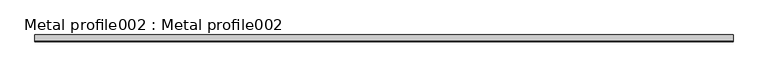
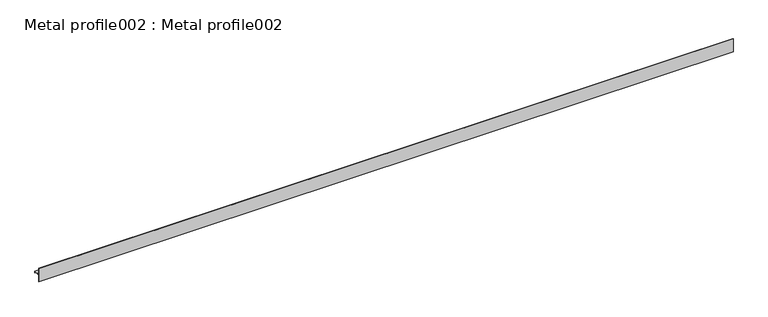
"""IFC4 building model written with IfcOpenShell, lengths in millimetres: proxy geometry, Metal profile002 : Metal profile002."""

from ifc_helpers import new_model, si_unit, frame, origin, place, context, project, spatial, polyline, outline, extrude, source, transform, mapped, element, save


def metal_profile002_metal_profile002_88e4c6c3(model_context):
    return source(origin(), model_context, "Body", "SweptSolid", [
        extrude(outline(polyline([(10460.9050834, 40757.6682813), (10443.9411354, 40757.6682813), (10443.9411354, 40738.6182812), (10442.6711354, 40738.6182812), (10442.6711354, 40777.9882813), (10443.9411354, 40777.9882813), (10443.9411354, 40758.9382813), (10462.1750834, 40758.9382813), (10462.1750834, 40754.1884812), (10460.9050834, 40754.1884812), (10460.9050834, 40757.6682813)])), frame((3694.2883192, 0.0, 0.0), z_axis=(1.0, 0.0, 0.0), x_axis=(0.0, 1.0, 0.0)), (0.0, 0.0, 1.0), 2000.0),
    ])


if __name__ == "__main__":
    model = new_model("IFC4")
    model_context = context("Model", 3, world=origin())
    ifc_project = project(units=[si_unit("LENGTHUNIT", "METRE", prefix="MILLI")], contexts=[model_context])
    site = spatial("IfcSite", under=ifc_project)
    building = spatial("IfcBuilding", under=site)
    placement = place(None, origin())
    metal_profile002_metal_profile002_shape = metal_profile002_metal_profile002_88e4c6c3(model_context)
    element("IfcBuildingElementProxy", 1, Name="Metal profile002 : Metal profile002", ObjectType="Metal profile002 : Metal profile002", at=placement, inside=building, context=model_context, shape_type="MappedRepresentation", body=[
        mapped(metal_profile002_metal_profile002_shape, transform((0.0, 0.0, 0.0), x_axis=(1.0, 0.0, 0.0), y_axis=(0.0, 1.0, 0.0), z_axis=(0.0, 0.0, 1.0))),
    ])
    save(model, "model.ifc")

# Revit data of these elements
# Type "Metal profile002 : Metal profile002"
#   NameOverride = "Metal profile002"
# Element 1 (IfcBuildingElementProxy, "Metal profile002 : Metal profile002")
#   Materials on its faces: "16 GA. COPPER VENTED T REVEAL BEAD"
# Materials
#   "16 GA. COPPER VENTED T REVEAL BEAD": class "Unassigned", colour RGB 255 227 10, transparency 0
